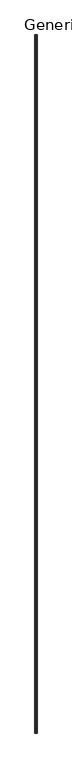
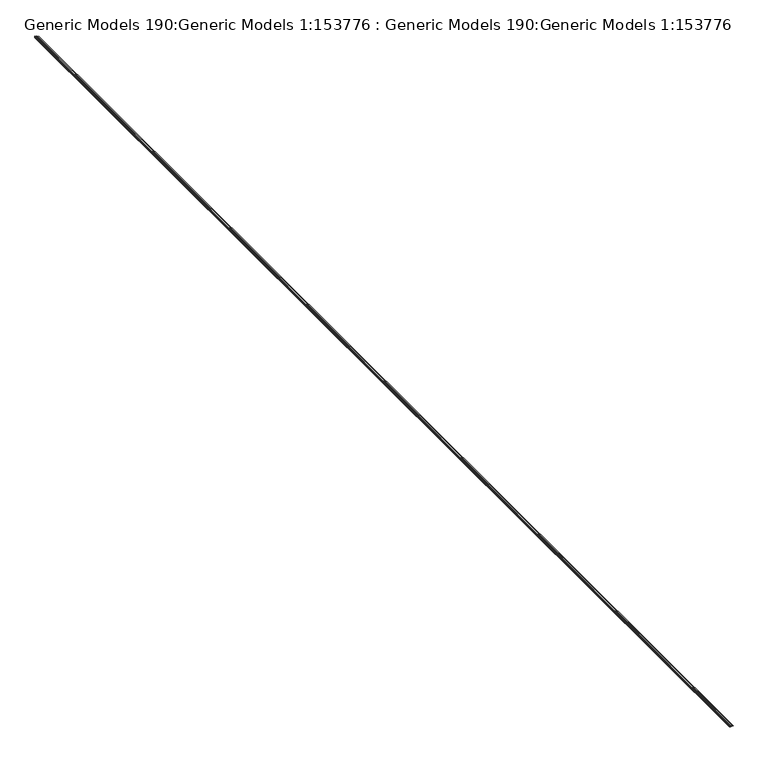
"""IFC4 building model written with IfcOpenShell, lengths in millimetres: proxy geometry, Generic Models 190:Generic Models 1:153776 : Generic Models 190:Generic Models 1:153776."""

import ifcopenshell
import ifcopenshell.guid

model = None  # the IFC model being written
_history = None  # IfcOwnerHistory: only IFC2X3 demands one
_inside = {}  # id of a spatial element -> (the spatial element, [elements in it])
_under = {}  # id of a project, library or spatial element -> (it, [spatial elements below it])
_declared = {}  # id of a project -> (the project, [libraries it declares])
_typed = {}  # id of a type object -> (the type object, [elements of that type])
_made_of = {}  # id of a material, layer set ... -> (it, [elements and type objects made of it])


def new_model(schema):
    """Start an empty IFC model of exactly this schema.

    Asked for "IFC4X3", IfcOpenShell would pick the latest addendum, in which some entities
    have other attributes; the version numbers below select the first issue.
    IFC2X3 requires an IfcOwnerHistory on every rooted entity: one is made here for all.
    """
    global model, _history
    if schema == "IFC4X3":
        model = ifcopenshell.file(schema_version=(4, 3, 0, 0))
    else:
        model = ifcopenshell.file(schema=schema)
    _inside.clear()
    _under.clear()
    _declared.clear()
    _typed.clear()
    _made_of.clear()
    _history = None
    if model.schema == "IFC2X3":
        org = make("IfcOrganization", Name="unknown")
        user = make(
            "IfcPersonAndOrganization",
            ThePerson=make("IfcPerson", FamilyName="unknown"),
            TheOrganization=org,
        )
        app = make(
            "IfcApplication",
            ApplicationDeveloper=org,
            Version="unknown",
            ApplicationFullName="unknown",
            ApplicationIdentifier="unknown",
        )
        _history = make(
            "IfcOwnerHistory",
            OwningUser=user,
            OwningApplication=app,
            ChangeAction="ADDED",
            CreationDate=0,
        )
    return model


def make(cls, **values):
    """One entity of the class cls with the attributes given. An attribute that is None is left unset."""
    return model.create_entity(
        cls, **{name: value for name, value in values.items() if value is not None}
    )


def rooted(cls, **values):
    """An entity with a GlobalId (a new one), such as an element, a storey or a relation."""
    return make(cls, GlobalId=ifcopenshell.guid.new(), OwnerHistory=_history, **values)


def si_unit(unit_type, name, prefix=None):
    """IfcSIUnit, for example si_unit("LENGTHUNIT", "METRE", prefix="MILLI")."""
    return make("IfcSIUnit", UnitType=unit_type, Prefix=prefix, Name=name)


def assignment(units):
    """IfcUnitAssignment: the units of a project."""
    return None if units is None else make("IfcUnitAssignment", Units=units)


def point(xyz):
    """IfcCartesianPoint."""
    return None if xyz is None else make("IfcCartesianPoint", Coordinates=xyz)


def direction(xyz):
    """IfcDirection."""
    return None if xyz is None else make("IfcDirection", DirectionRatios=xyz)


def frame(location, z_axis=None, x_axis=None):
    """IfcAxis2Placement3D, a coordinate frame: its origin and axes. An axis left out is left unset."""
    return make(
        "IfcAxis2Placement3D",
        Location=point(location),
        Axis=direction(z_axis),
        RefDirection=direction(x_axis),
    )


def origin():
    """The frame at (0, 0, 0) with its axes left unset."""
    return frame((0.0, 0.0, 0.0))


def place(relative_to, where):
    """IfcLocalPlacement: puts the frame where relative to a parent placement (None: the world)."""
    return make(
        "IfcLocalPlacement", PlacementRelTo=relative_to, RelativePlacement=where
    )


def context(
    kind, dimensions, precision=None, world=None, true_north=None, identifier=None
):
    """IfcGeometricRepresentationContext, for example the 3D "Model" context."""
    return make(
        "IfcGeometricRepresentationContext",
        ContextIdentifier=identifier,
        ContextType=kind,
        CoordinateSpaceDimension=dimensions,
        Precision=precision,
        WorldCoordinateSystem=world,
        TrueNorth=true_north,
    )


def project(units=None, contexts=None):
    """IfcProject with its units and contexts."""
    return rooted(
        "IfcProject",
        Name="project",
        RepresentationContexts=contexts,
        UnitsInContext=assignment(units),
    )


def spatial(cls, under=None, at=None, **own):
    """A site, building, storey or space (cls), placed at a placement, below another one or the project."""
    s = rooted(cls, ObjectPlacement=at, **own)
    if under is not None:
        _under.setdefault(under.id(), (under, []))[1].append(s)
    return s


def polyline(points):
    """IfcPolyline through the points."""
    return make("IfcPolyline", Points=[point(p) for p in points])


def outline(outer, holes=None, kind="AREA"):
    """IfcArbitraryClosedProfileDef: a profile drawn as a closed curve; with holes, ...WithVoids."""
    if holes is None:
        return make("IfcArbitraryClosedProfileDef", ProfileType=kind, OuterCurve=outer)
    return make(
        "IfcArbitraryProfileDefWithVoids",
        ProfileType=kind,
        OuterCurve=outer,
        InnerCurves=holes,
    )


def extrude(swept, where, along, depth):
    """IfcExtrudedAreaSolid: the profile swept, set in the frame where, extruded along a direction by depth."""
    return make(
        "IfcExtrudedAreaSolid",
        SweptArea=swept,
        Position=where,
        ExtrudedDirection=direction(along),
        Depth=depth,
    )


def shape(context_of_items, identifier, shape_type, items):
    """IfcShapeRepresentation: the items that make up one representation, for example the "Body"."""
    return make(
        "IfcShapeRepresentation",
        ContextOfItems=context_of_items,
        RepresentationIdentifier=identifier,
        RepresentationType=shape_type,
        Items=items,
    )


def source(mapping_origin, context_of_items, identifier, shape_type, items):
    """IfcRepresentationMap: a shape defined once, which mapped items show again and again."""
    return make(
        "IfcRepresentationMap",
        MappingOrigin=mapping_origin,
        MappedRepresentation=shape(context_of_items, identifier, shape_type, items),
    )


def transform(
    local_origin,
    x_axis=None,
    y_axis=None,
    z_axis=None,
    scale=None,
    scale2=None,
    scale3=None,
    uniform=True,
):
    """IfcCartesianTransformationOperator3D, or its non-uniform kind. x_axis, y_axis, z_axis: its Axis1, 2, 3."""
    if uniform:
        return make(
            "IfcCartesianTransformationOperator3D",
            Axis1=direction(x_axis),
            Axis2=direction(y_axis),
            LocalOrigin=point(local_origin),
            Scale=scale,
            Axis3=direction(z_axis),
        )
    return make(
        "IfcCartesianTransformationOperator3DnonUniform",
        Axis1=direction(x_axis),
        Axis2=direction(y_axis),
        LocalOrigin=point(local_origin),
        Scale=scale,
        Axis3=direction(z_axis),
        Scale2=scale2,
        Scale3=scale3,
    )


def mapped(mapping_source, mapping_target):
    """IfcMappedItem: shows the shape of a source again, moved by a transform."""
    return make(
        "IfcMappedItem", MappingSource=mapping_source, MappingTarget=mapping_target
    )


def made_of(thing, what):
    """Note that an element or type object is made of a material, layer set ...; save() writes the relation."""
    if what is not None:
        _made_of.setdefault(what.id(), (what, []))[1].append(thing)
    return thing


def element(
    cls,
    number,
    at=None,
    inside=None,
    cuts=None,
    type_object=None,
    material=None,
    context=None,
    identifier="Body",
    shape_type=None,
    held_by="IfcProductDefinitionShape",
    body=None,
    shapes=None,
    **own,
):
    """One element of the class cls, such as IfcWall. Its Tag is "e" and its number.

    at: its placement. inside: the storey or other place that contains it. cuts: it is an
    opening in that element (IfcRelVoidsElement). A single representation is given by context,
    identifier, shape_type and body (its items); several are given by shapes. held_by: the class
    of the entity that holds the representations. save() writes the other relations.
    """
    e = rooted(cls, Tag="e%d" % number, ObjectPlacement=at, **own)
    if body is not None:
        shapes = [shape(context, identifier, shape_type, body)]
    if shapes is not None:
        e.Representation = make(held_by, Representations=shapes)
    if inside is not None:
        _inside.setdefault(inside.id(), (inside, []))[1].append(e)
    if cuts is not None:
        rooted(
            "IfcRelVoidsElement", RelatingBuildingElement=cuts, RelatedOpeningElement=e
        )
    if type_object is not None:
        _typed.setdefault(type_object.id(), (type_object, []))[1].append(e)
    return made_of(e, material)


def aggregate(whole, parts):
    """IfcRelAggregates: a whole, such as a stair, and the parts it consists of."""
    return rooted("IfcRelAggregates", RelatingObject=whole, RelatedObjects=parts)


def save(model, path):
    """Write the relations noted so far, then the file.

    IfcRelAggregates (storeys below a building ...), IfcRelContainedInSpatialStructure (elements
    in a storey), IfcRelDefinesByType, IfcRelAssociatesMaterial and IfcRelDeclares: one each for
    every whole, place, type object, material and project.
    """
    for whole, parts in _under.values():
        aggregate(whole, parts)
    for where, things in _inside.values():
        rooted(
            "IfcRelContainedInSpatialStructure",
            RelatedElements=things,
            RelatingStructure=where,
        )
    for kind, things in _typed.values():
        rooted("IfcRelDefinesByType", RelatedObjects=things, RelatingType=kind)
    for what, things in _made_of.values():
        rooted("IfcRelAssociatesMaterial", RelatedObjects=things, RelatingMaterial=what)
    for by, libraries in _declared.values():
        rooted("IfcRelDeclares", RelatingContext=by, RelatedDefinitions=libraries)
    model.write(path)


def generic_models_190_generic_models_1_153776_generic_models_7bb808aa(model_context):
    return source(origin(), model_context, "Body", "SweptSolid", [
        extrude(outline(polyline([(5932.0389027, -5376.1243913), (5932.0389027, -5395.8093913), (5934.2487027, -5395.8093913), (5934.2487027, -5394.9505504), (5954.5632814, -5394.9505504), (5954.5632814, -5396.2205504), (5935.5187027, -5396.2205504), (5935.5187027, -5397.0793913), (5930.7689027, -5397.0793913), (5930.7689027, -5374.8543913), (5942.1989027, -5374.8543913), (5942.1989027, -5362.1543913), (5930.7689027, -5362.1543913), (5930.7689027, -5338.4412074), (5932.0389027, -5338.4412074), (5932.0389027, -5360.8843913), (5943.4689027, -5360.8843913), (5943.4689027, -5376.1243913), (5932.0389027, -5376.1243913)])), frame((0.0, -6877.9974793, 0.0), z_axis=(0.0, 1.0, 0.0), x_axis=(0.0, 0.0, 1.0)), (0.0, 0.0, 1.0), 19050.0),
    ])


if __name__ == "__main__":
    model = new_model("IFC4")
    model_context = context("Model", 3, world=origin())
    ifc_project = project(units=[si_unit("LENGTHUNIT", "METRE", prefix="MILLI")], contexts=[model_context])
    site = spatial("IfcSite", under=ifc_project)
    building = spatial("IfcBuilding", under=site)
    placement = place(None, origin())
    generic_models_190_generic_models_1_153776_generic_models_shape = generic_models_190_generic_models_1_153776_generic_models_7bb808aa(model_context)
    element("IfcBuildingElementProxy", 1, Name="Generic Models 190:Generic Models 1:153776 : Generic Models 190:Generic Models 1:153776", ObjectType="Generic Models 190:Generic Models 1:153776 : Generic Models 190:Generic Models 1:153776", at=placement, inside=building, context=model_context, shape_type="MappedRepresentation", body=[
        mapped(generic_models_190_generic_models_1_153776_generic_models_shape, transform((0.0, 0.0, 0.0), x_axis=(1.0, 0.0, 0.0), y_axis=(0.0, 1.0, 0.0), z_axis=(0.0, 0.0, 1.0))),
    ])
    save(model, "model.ifc")

# Revit data of these elements
# Type "Generic Models 190:Generic Models 1:153776 : Generic Models 190:Generic Models 1:153776"
#   NameOverride = "Generic Models 190:Generic Models 1:153776"
#   ObjectTypeOverride = "Generic Models 190:Generic Models 1"
#   Reference = "Generic Models 1"
#   Category = "Generic Models"
#   Tag = "153776"
# Element 1 (IfcBuildingElementProxy, "Generic Models 190:Generic Models 1:153776 : Generic Models 190:Generic Models 1:153776")
#   Materials on its faces: "_16 GA. COPPER SOFFIT DRIP SCREED 1359"
# Materials
#   "_16 GA. COPPER SOFFIT DRIP SCREED 1359": class "Unassigned", colour RGB 253 192 103, transparency 0
